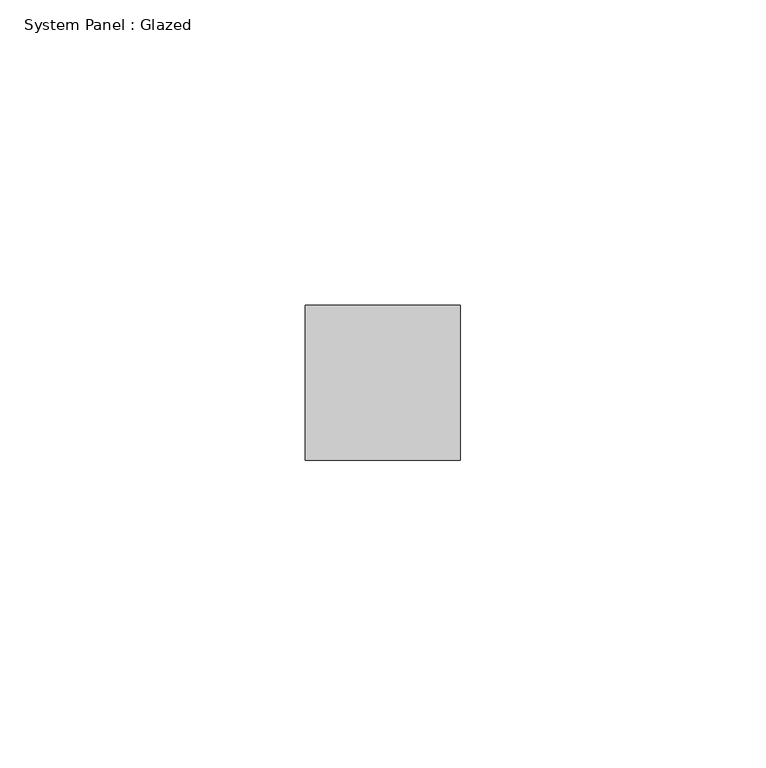
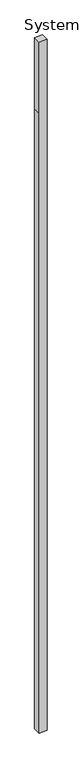
"""IFC4 building model written with IfcOpenShell, lengths in millimetres: plate geometry, System Panel : Glazed."""

import ifcopenshell
import ifcopenshell.guid

model = None  # the IFC model being written
_history = None  # IfcOwnerHistory: only IFC2X3 demands one
_inside = {}  # id of a spatial element -> (the spatial element, [elements in it])
_under = {}  # id of a project, library or spatial element -> (it, [spatial elements below it])
_declared = {}  # id of a project -> (the project, [libraries it declares])
_typed = {}  # id of a type object -> (the type object, [elements of that type])
_made_of = {}  # id of a material, layer set ... -> (it, [elements and type objects made of it])


def new_model(schema):
    """Start an empty IFC model of exactly this schema.

    Asked for "IFC4X3", IfcOpenShell would pick the latest addendum, in which some entities
    have other attributes; the version numbers below select the first issue.
    IFC2X3 requires an IfcOwnerHistory on every rooted entity: one is made here for all.
    """
    global model, _history
    if schema == "IFC4X3":
        model = ifcopenshell.file(schema_version=(4, 3, 0, 0))
    else:
        model = ifcopenshell.file(schema=schema)
    _inside.clear()
    _under.clear()
    _declared.clear()
    _typed.clear()
    _made_of.clear()
    _history = None
    if model.schema == "IFC2X3":
        org = make("IfcOrganization", Name="unknown")
        user = make(
            "IfcPersonAndOrganization",
            ThePerson=make("IfcPerson", FamilyName="unknown"),
            TheOrganization=org,
        )
        app = make(
            "IfcApplication",
            ApplicationDeveloper=org,
            Version="unknown",
            ApplicationFullName="unknown",
            ApplicationIdentifier="unknown",
        )
        _history = make(
            "IfcOwnerHistory",
            OwningUser=user,
            OwningApplication=app,
            ChangeAction="ADDED",
            CreationDate=0,
        )
    return model


def make(cls, **values):
    """One entity of the class cls with the attributes given. An attribute that is None is left unset."""
    return model.create_entity(
        cls, **{name: value for name, value in values.items() if value is not None}
    )


def rooted(cls, **values):
    """An entity with a GlobalId (a new one), such as an element, a storey or a relation."""
    return make(cls, GlobalId=ifcopenshell.guid.new(), OwnerHistory=_history, **values)


def si_unit(unit_type, name, prefix=None):
    """IfcSIUnit, for example si_unit("LENGTHUNIT", "METRE", prefix="MILLI")."""
    return make("IfcSIUnit", UnitType=unit_type, Prefix=prefix, Name=name)


def assignment(units):
    """IfcUnitAssignment: the units of a project."""
    return None if units is None else make("IfcUnitAssignment", Units=units)


def point(xyz):
    """IfcCartesianPoint."""
    return None if xyz is None else make("IfcCartesianPoint", Coordinates=xyz)


def direction(xyz):
    """IfcDirection."""
    return None if xyz is None else make("IfcDirection", DirectionRatios=xyz)


def frame(location, z_axis=None, x_axis=None):
    """IfcAxis2Placement3D, a coordinate frame: its origin and axes. An axis left out is left unset."""
    return make(
        "IfcAxis2Placement3D",
        Location=point(location),
        Axis=direction(z_axis),
        RefDirection=direction(x_axis),
    )


def origin():
    """The frame at (0, 0, 0) with its axes left unset."""
    return frame((0.0, 0.0, 0.0))


def place(relative_to, where):
    """IfcLocalPlacement: puts the frame where relative to a parent placement (None: the world)."""
    return make(
        "IfcLocalPlacement", PlacementRelTo=relative_to, RelativePlacement=where
    )


def context(
    kind, dimensions, precision=None, world=None, true_north=None, identifier=None
):
    """IfcGeometricRepresentationContext, for example the 3D "Model" context."""
    return make(
        "IfcGeometricRepresentationContext",
        ContextIdentifier=identifier,
        ContextType=kind,
        CoordinateSpaceDimension=dimensions,
        Precision=precision,
        WorldCoordinateSystem=world,
        TrueNorth=true_north,
    )


def project(units=None, contexts=None):
    """IfcProject with its units and contexts."""
    return rooted(
        "IfcProject",
        Name="project",
        RepresentationContexts=contexts,
        UnitsInContext=assignment(units),
    )


def spatial(cls, under=None, at=None, **own):
    """A site, building, storey or space (cls), placed at a placement, below another one or the project."""
    s = rooted(cls, ObjectPlacement=at, **own)
    if under is not None:
        _under.setdefault(under.id(), (under, []))[1].append(s)
    return s


def polyline(points):
    """IfcPolyline through the points."""
    return make("IfcPolyline", Points=[point(p) for p in points])


def outline(outer, holes=None, kind="AREA"):
    """IfcArbitraryClosedProfileDef: a profile drawn as a closed curve; with holes, ...WithVoids."""
    if holes is None:
        return make("IfcArbitraryClosedProfileDef", ProfileType=kind, OuterCurve=outer)
    return make(
        "IfcArbitraryProfileDefWithVoids",
        ProfileType=kind,
        OuterCurve=outer,
        InnerCurves=holes,
    )


def extrude(swept, where, along, depth):
    """IfcExtrudedAreaSolid: the profile swept, set in the frame where, extruded along a direction by depth."""
    return make(
        "IfcExtrudedAreaSolid",
        SweptArea=swept,
        Position=where,
        ExtrudedDirection=direction(along),
        Depth=depth,
    )


def shape(context_of_items, identifier, shape_type, items):
    """IfcShapeRepresentation: the items that make up one representation, for example the "Body"."""
    return make(
        "IfcShapeRepresentation",
        ContextOfItems=context_of_items,
        RepresentationIdentifier=identifier,
        RepresentationType=shape_type,
        Items=items,
    )


def source(mapping_origin, context_of_items, identifier, shape_type, items):
    """IfcRepresentationMap: a shape defined once, which mapped items show again and again."""
    return make(
        "IfcRepresentationMap",
        MappingOrigin=mapping_origin,
        MappedRepresentation=shape(context_of_items, identifier, shape_type, items),
    )


def transform(
    local_origin,
    x_axis=None,
    y_axis=None,
    z_axis=None,
    scale=None,
    scale2=None,
    scale3=None,
    uniform=True,
):
    """IfcCartesianTransformationOperator3D, or its non-uniform kind. x_axis, y_axis, z_axis: its Axis1, 2, 3."""
    if uniform:
        return make(
            "IfcCartesianTransformationOperator3D",
            Axis1=direction(x_axis),
            Axis2=direction(y_axis),
            LocalOrigin=point(local_origin),
            Scale=scale,
            Axis3=direction(z_axis),
        )
    return make(
        "IfcCartesianTransformationOperator3DnonUniform",
        Axis1=direction(x_axis),
        Axis2=direction(y_axis),
        LocalOrigin=point(local_origin),
        Scale=scale,
        Axis3=direction(z_axis),
        Scale2=scale2,
        Scale3=scale3,
    )


def mapped(mapping_source, mapping_target):
    """IfcMappedItem: shows the shape of a source again, moved by a transform."""
    return make(
        "IfcMappedItem", MappingSource=mapping_source, MappingTarget=mapping_target
    )


def made_of(thing, what):
    """Note that an element or type object is made of a material, layer set ...; save() writes the relation."""
    if what is not None:
        _made_of.setdefault(what.id(), (what, []))[1].append(thing)
    return thing


def element(
    cls,
    number,
    at=None,
    inside=None,
    cuts=None,
    type_object=None,
    material=None,
    context=None,
    identifier="Body",
    shape_type=None,
    held_by="IfcProductDefinitionShape",
    body=None,
    shapes=None,
    **own,
):
    """One element of the class cls, such as IfcWall. Its Tag is "e" and its number.

    at: its placement. inside: the storey or other place that contains it. cuts: it is an
    opening in that element (IfcRelVoidsElement). A single representation is given by context,
    identifier, shape_type and body (its items); several are given by shapes. held_by: the class
    of the entity that holds the representations. save() writes the other relations.
    """
    e = rooted(cls, Tag="e%d" % number, ObjectPlacement=at, **own)
    if body is not None:
        shapes = [shape(context, identifier, shape_type, body)]
    if shapes is not None:
        e.Representation = make(held_by, Representations=shapes)
    if inside is not None:
        _inside.setdefault(inside.id(), (inside, []))[1].append(e)
    if cuts is not None:
        rooted(
            "IfcRelVoidsElement", RelatingBuildingElement=cuts, RelatedOpeningElement=e
        )
    if type_object is not None:
        _typed.setdefault(type_object.id(), (type_object, []))[1].append(e)
    return made_of(e, material)


def aggregate(whole, parts):
    """IfcRelAggregates: a whole, such as a stair, and the parts it consists of."""
    return rooted("IfcRelAggregates", RelatingObject=whole, RelatedObjects=parts)


def save(model, path):
    """Write the relations noted so far, then the file.

    IfcRelAggregates (storeys below a building ...), IfcRelContainedInSpatialStructure (elements
    in a storey), IfcRelDefinesByType, IfcRelAssociatesMaterial and IfcRelDeclares: one each for
    every whole, place, type object, material and project.
    """
    for whole, parts in _under.values():
        aggregate(whole, parts)
    for where, things in _inside.values():
        rooted(
            "IfcRelContainedInSpatialStructure",
            RelatedElements=things,
            RelatingStructure=where,
        )
    for kind, things in _typed.values():
        rooted("IfcRelDefinesByType", RelatedObjects=things, RelatingType=kind)
    for what, things in _made_of.values():
        rooted("IfcRelAssociatesMaterial", RelatedObjects=things, RelatingMaterial=what)
    for by, libraries in _declared.values():
        rooted("IfcRelDeclares", RelatingContext=by, RelatedDefinitions=libraries)
    model.write(path)


def system_panel_glazed_99e16266(model_context):
    return source(origin(), model_context, "Body", "SweptSolid", [
        extrude(outline(polyline([(0.0, -12.7), (0.0, 12.7), (2101.85, 12.7), (2343.15, 12.7), (2343.15, -12.7), (2101.85, -12.7), (0.0, -12.7)])), frame((0.0, 19.05, 0.0), z_axis=(0.0, 1.0, 0.0), x_axis=(0.0, 0.0, 1.0)), (0.0, 0.0, 1.0), 25.4),
    ])


if __name__ == "__main__":
    model = new_model("IFC4")
    model_context = context("Model", 3, world=origin())
    ifc_project = project(units=[si_unit("LENGTHUNIT", "METRE", prefix="MILLI")], contexts=[model_context])
    site = spatial("IfcSite", under=ifc_project)
    building = spatial("IfcBuilding", under=site)
    placement = place(None, origin())
    system_panel_glazed_shape = system_panel_glazed_99e16266(model_context)
    element("IfcPlate", 1, ObjectType="System Panel : Glazed", at=placement, inside=building, context=model_context, shape_type="MappedRepresentation", body=[
        mapped(system_panel_glazed_shape, transform((0.0, 0.0, 0.0), x_axis=(1.0, 0.0, 0.0), y_axis=(0.0, 1.0, 0.0), z_axis=(0.0, 0.0, 1.0))),
    ])
    save(model, "model.ifc")

# Revit data of these elements
# Element 1 (IfcPlate, "System Panel : Glazed")
#   Materials on its faces: "Glass"
# Materials
#   "Glass": class "Glass", colour RGB 0 128 192, transparency 0.75
